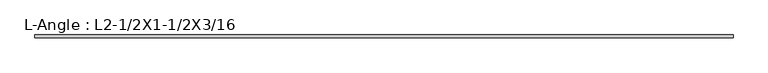
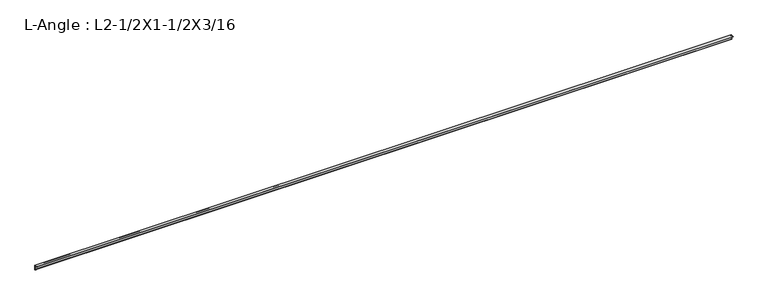
"""IFC4 building model written with IfcOpenShell, lengths in millimetres: beam geometry, L-Angle : L2-1/2X1-1/2X3/16."""

import ifcopenshell
import ifcopenshell.guid

model = None  # the IFC model being written
_history = None  # IfcOwnerHistory: only IFC2X3 demands one
_inside = {}  # id of a spatial element -> (the spatial element, [elements in it])
_under = {}  # id of a project, library or spatial element -> (it, [spatial elements below it])
_declared = {}  # id of a project -> (the project, [libraries it declares])
_typed = {}  # id of a type object -> (the type object, [elements of that type])
_made_of = {}  # id of a material, layer set ... -> (it, [elements and type objects made of it])


def new_model(schema):
    """Start an empty IFC model of exactly this schema.

    Asked for "IFC4X3", IfcOpenShell would pick the latest addendum, in which some entities
    have other attributes; the version numbers below select the first issue.
    IFC2X3 requires an IfcOwnerHistory on every rooted entity: one is made here for all.
    """
    global model, _history
    if schema == "IFC4X3":
        model = ifcopenshell.file(schema_version=(4, 3, 0, 0))
    else:
        model = ifcopenshell.file(schema=schema)
    _inside.clear()
    _under.clear()
    _declared.clear()
    _typed.clear()
    _made_of.clear()
    _history = None
    if model.schema == "IFC2X3":
        org = make("IfcOrganization", Name="unknown")
        user = make(
            "IfcPersonAndOrganization",
            ThePerson=make("IfcPerson", FamilyName="unknown"),
            TheOrganization=org,
        )
        app = make(
            "IfcApplication",
            ApplicationDeveloper=org,
            Version="unknown",
            ApplicationFullName="unknown",
            ApplicationIdentifier="unknown",
        )
        _history = make(
            "IfcOwnerHistory",
            OwningUser=user,
            OwningApplication=app,
            ChangeAction="ADDED",
            CreationDate=0,
        )
    return model


def make(cls, **values):
    """One entity of the class cls with the attributes given. An attribute that is None is left unset."""
    return model.create_entity(
        cls, **{name: value for name, value in values.items() if value is not None}
    )


def rooted(cls, **values):
    """An entity with a GlobalId (a new one), such as an element, a storey or a relation."""
    return make(cls, GlobalId=ifcopenshell.guid.new(), OwnerHistory=_history, **values)


def si_unit(unit_type, name, prefix=None):
    """IfcSIUnit, for example si_unit("LENGTHUNIT", "METRE", prefix="MILLI")."""
    return make("IfcSIUnit", UnitType=unit_type, Prefix=prefix, Name=name)


def assignment(units):
    """IfcUnitAssignment: the units of a project."""
    return None if units is None else make("IfcUnitAssignment", Units=units)


def point(xyz):
    """IfcCartesianPoint."""
    return None if xyz is None else make("IfcCartesianPoint", Coordinates=xyz)


def direction(xyz):
    """IfcDirection."""
    return None if xyz is None else make("IfcDirection", DirectionRatios=xyz)


def frame(location, z_axis=None, x_axis=None):
    """IfcAxis2Placement3D, a coordinate frame: its origin and axes. An axis left out is left unset."""
    return make(
        "IfcAxis2Placement3D",
        Location=point(location),
        Axis=direction(z_axis),
        RefDirection=direction(x_axis),
    )


def frame_2d(location, x_axis=None):
    """IfcAxis2Placement2D, a coordinate frame in the plane: its origin and x axis."""
    return make(
        "IfcAxis2Placement2D", Location=point(location), RefDirection=direction(x_axis)
    )


def origin():
    """The frame at (0, 0, 0) with its axes left unset."""
    return frame((0.0, 0.0, 0.0))


def place(relative_to, where):
    """IfcLocalPlacement: puts the frame where relative to a parent placement (None: the world)."""
    return make(
        "IfcLocalPlacement", PlacementRelTo=relative_to, RelativePlacement=where
    )


def context(
    kind, dimensions, precision=None, world=None, true_north=None, identifier=None
):
    """IfcGeometricRepresentationContext, for example the 3D "Model" context."""
    return make(
        "IfcGeometricRepresentationContext",
        ContextIdentifier=identifier,
        ContextType=kind,
        CoordinateSpaceDimension=dimensions,
        Precision=precision,
        WorldCoordinateSystem=world,
        TrueNorth=true_north,
    )


def project(units=None, contexts=None):
    """IfcProject with its units and contexts."""
    return rooted(
        "IfcProject",
        Name="project",
        RepresentationContexts=contexts,
        UnitsInContext=assignment(units),
    )


def spatial(cls, under=None, at=None, **own):
    """A site, building, storey or space (cls), placed at a placement, below another one or the project."""
    s = rooted(cls, ObjectPlacement=at, **own)
    if under is not None:
        _under.setdefault(under.id(), (under, []))[1].append(s)
    return s


def polyline(points):
    """IfcPolyline through the points."""
    return make("IfcPolyline", Points=[point(p) for p in points])


def circle_curve(where, radius):
    """IfcCircle in the frame where."""
    return make("IfcCircle", Position=where, Radius=radius)


def trimmed(basis, trim1, trim2, sense, master):
    """IfcTrimmedCurve: the piece of a basis curve between two trims."""
    return make(
        "IfcTrimmedCurve",
        BasisCurve=basis,
        Trim1=trim1,
        Trim2=trim2,
        SenseAgreement=sense,
        MasterRepresentation=master,
    )


def segment(curve, same_sense, transition):
    """IfcCompositeCurveSegment."""
    return make(
        "IfcCompositeCurveSegment",
        Transition=transition,
        SameSense=same_sense,
        ParentCurve=curve,
    )


def composite_curve(segments, self_intersect=None):
    """IfcCompositeCurve: segments joined end to end."""
    return make("IfcCompositeCurve", Segments=segments, SelfIntersect=self_intersect)


def outline(outer, holes=None, kind="AREA"):
    """IfcArbitraryClosedProfileDef: a profile drawn as a closed curve; with holes, ...WithVoids."""
    if holes is None:
        return make("IfcArbitraryClosedProfileDef", ProfileType=kind, OuterCurve=outer)
    return make(
        "IfcArbitraryProfileDefWithVoids",
        ProfileType=kind,
        OuterCurve=outer,
        InnerCurves=holes,
    )


def extrude(swept, where, along, depth):
    """IfcExtrudedAreaSolid: the profile swept, set in the frame where, extruded along a direction by depth."""
    return make(
        "IfcExtrudedAreaSolid",
        SweptArea=swept,
        Position=where,
        ExtrudedDirection=direction(along),
        Depth=depth,
    )


def shape(context_of_items, identifier, shape_type, items):
    """IfcShapeRepresentation: the items that make up one representation, for example the "Body"."""
    return make(
        "IfcShapeRepresentation",
        ContextOfItems=context_of_items,
        RepresentationIdentifier=identifier,
        RepresentationType=shape_type,
        Items=items,
    )


def source(mapping_origin, context_of_items, identifier, shape_type, items):
    """IfcRepresentationMap: a shape defined once, which mapped items show again and again."""
    return make(
        "IfcRepresentationMap",
        MappingOrigin=mapping_origin,
        MappedRepresentation=shape(context_of_items, identifier, shape_type, items),
    )


def transform(
    local_origin,
    x_axis=None,
    y_axis=None,
    z_axis=None,
    scale=None,
    scale2=None,
    scale3=None,
    uniform=True,
):
    """IfcCartesianTransformationOperator3D, or its non-uniform kind. x_axis, y_axis, z_axis: its Axis1, 2, 3."""
    if uniform:
        return make(
            "IfcCartesianTransformationOperator3D",
            Axis1=direction(x_axis),
            Axis2=direction(y_axis),
            LocalOrigin=point(local_origin),
            Scale=scale,
            Axis3=direction(z_axis),
        )
    return make(
        "IfcCartesianTransformationOperator3DnonUniform",
        Axis1=direction(x_axis),
        Axis2=direction(y_axis),
        LocalOrigin=point(local_origin),
        Scale=scale,
        Axis3=direction(z_axis),
        Scale2=scale2,
        Scale3=scale3,
    )


def mapped(mapping_source, mapping_target):
    """IfcMappedItem: shows the shape of a source again, moved by a transform."""
    return make(
        "IfcMappedItem", MappingSource=mapping_source, MappingTarget=mapping_target
    )


def made_of(thing, what):
    """Note that an element or type object is made of a material, layer set ...; save() writes the relation."""
    if what is not None:
        _made_of.setdefault(what.id(), (what, []))[1].append(thing)
    return thing


def element(
    cls,
    number,
    at=None,
    inside=None,
    cuts=None,
    type_object=None,
    material=None,
    context=None,
    identifier="Body",
    shape_type=None,
    held_by="IfcProductDefinitionShape",
    body=None,
    shapes=None,
    **own,
):
    """One element of the class cls, such as IfcWall. Its Tag is "e" and its number.

    at: its placement. inside: the storey or other place that contains it. cuts: it is an
    opening in that element (IfcRelVoidsElement). A single representation is given by context,
    identifier, shape_type and body (its items); several are given by shapes. held_by: the class
    of the entity that holds the representations. save() writes the other relations.
    """
    e = rooted(cls, Tag="e%d" % number, ObjectPlacement=at, **own)
    if body is not None:
        shapes = [shape(context, identifier, shape_type, body)]
    if shapes is not None:
        e.Representation = make(held_by, Representations=shapes)
    if inside is not None:
        _inside.setdefault(inside.id(), (inside, []))[1].append(e)
    if cuts is not None:
        rooted(
            "IfcRelVoidsElement", RelatingBuildingElement=cuts, RelatedOpeningElement=e
        )
    if type_object is not None:
        _typed.setdefault(type_object.id(), (type_object, []))[1].append(e)
    return made_of(e, material)


def aggregate(whole, parts):
    """IfcRelAggregates: a whole, such as a stair, and the parts it consists of."""
    return rooted("IfcRelAggregates", RelatingObject=whole, RelatedObjects=parts)


def save(model, path):
    """Write the relations noted so far, then the file.

    IfcRelAggregates (storeys below a building ...), IfcRelContainedInSpatialStructure (elements
    in a storey), IfcRelDefinesByType, IfcRelAssociatesMaterial and IfcRelDeclares: one each for
    every whole, place, type object, material and project.
    """
    for whole, parts in _under.values():
        aggregate(whole, parts)
    for where, things in _inside.values():
        rooted(
            "IfcRelContainedInSpatialStructure",
            RelatedElements=things,
            RelatingStructure=where,
        )
    for kind, things in _typed.values():
        rooted("IfcRelDefinesByType", RelatedObjects=things, RelatingType=kind)
    for what, things in _made_of.values():
        rooted("IfcRelAssociatesMaterial", RelatedObjects=things, RelatingMaterial=what)
    for by, libraries in _declared.values():
        rooted("IfcRelDeclares", RelatingContext=by, RelatedDefinitions=libraries)
    model.write(path)


def l_angle_l2_1_2x1_1_2x3_16_b2e2aca2(model_context):
    return source(origin(), model_context, "Body", "SweptSolid", [
        extrude(outline(composite_curve([segment(polyline([(8.8138, 21.3106), (8.8138, -42.1894)]), True, "CONTINUOUS"), segment(trimmed(circle_curve(frame_2d((8.8138, -37.4269)), 4.7625), [point((8.8138, -42.1894))], [point((4.0513, -37.4269))], False, "CARTESIAN"), True, "CONTINUOUS"), segment(polyline([(4.0513, -37.4269), (4.0513, 11.7856)]), True, "CONTINUOUS"), segment(trimmed(circle_curve(frame_2d((-0.7112, 11.7856)), 4.7625), [point((4.0513, 11.7856))], [point((-0.7112, 16.5481))], True, "CARTESIAN"), True, "CONTINUOUS"), segment(polyline([(-0.7112, 16.5481), (-24.5237, 16.5481)]), True, "CONTINUOUS"), segment(trimmed(circle_curve(frame_2d((-24.5237, 21.3106)), 4.7625), [point((-24.5237, 16.5481))], [point((-29.2862, 21.3106))], False, "CARTESIAN"), True, "CONTINUOUS"), segment(polyline([(-29.2862, 21.3106), (8.8138, 21.3106)]), True, "CONTINUOUS")], self_intersect=False)), frame((-4623.1464888, 0.0, 0.0), z_axis=(1.0, 0.0, 0.0), x_axis=(0.0, 1.0, 0.0)), (0.0, 0.0, 1.0), 9512.5543207),
    ])


if __name__ == "__main__":
    model = new_model("IFC4")
    model_context = context("Model", 3, world=origin())
    ifc_project = project(units=[si_unit("LENGTHUNIT", "METRE", prefix="MILLI")], contexts=[model_context])
    site = spatial("IfcSite", under=ifc_project)
    building = spatial("IfcBuilding", under=site)
    placement = place(None, origin())
    l_angle_l2_1_2x1_1_2x3_16_shape = l_angle_l2_1_2x1_1_2x3_16_b2e2aca2(model_context)
    element("IfcBeam", 1, ObjectType="L-Angle : L2-1/2X1-1/2X3/16", at=placement, inside=building, context=model_context, shape_type="MappedRepresentation", body=[
        mapped(l_angle_l2_1_2x1_1_2x3_16_shape, transform((0.0, 0.0, 0.0), x_axis=(1.0, 0.0, 0.0), y_axis=(0.0, 1.0, 0.0), z_axis=(0.0, 0.0, 1.0))),
    ])
    save(model, "model.ifc")

# Revit data of these elements
# Type "L-Angle : L2-1/2X1-1/2X3/16"
#   Assembly Code = "B10"
#   k = 0' - 0 7/16"
#   W = 2.47
#   Start Extension Calculation [instance default] = 10' - 0"
#   Start Extension [instance default] = -0' - 0 1/2"
#   End Extension Calculation [instance default] = 10' - 0"
#   End Extension [instance default] = -0' - 0 1/2"
#   Length [instance default] = 5' - 0"
#   b = 0' - 1 1/2"
#   d = 0' - 2 1/2"
#   t = 0' - 0 3/16"
#   x = 0' - 0.347"
#   y = 0' - 0.839"
#   A = 0.00496528 SF
#   Structural Material [instance default] = Metal - Steel - ASTM A36
# Element 1 (IfcBeam, "L-Angle : L2-1/2X1-1/2X3/16")
#   Materials on its faces: "Metal - Steel - ASTM A36"
# Materials
#   "Metal - Steel - ASTM A36": class "Metal", colour RGB 199 199 199, transparency 0
